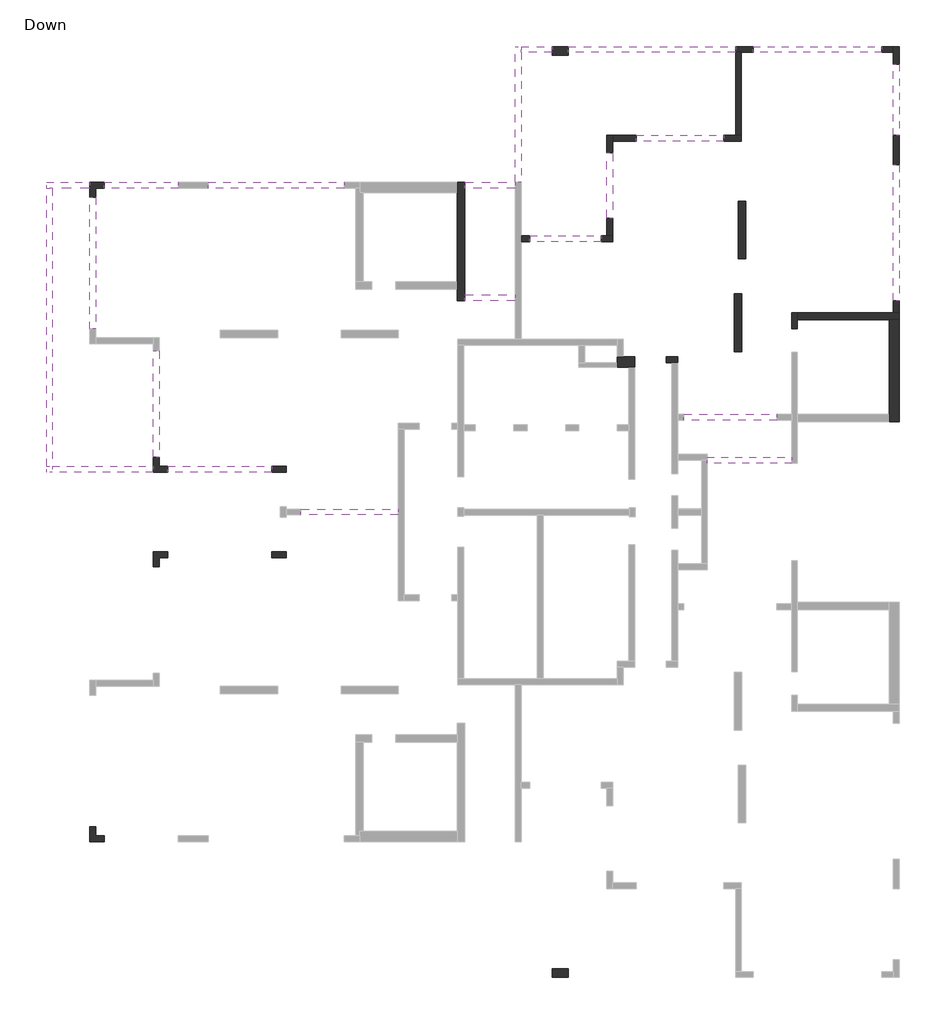
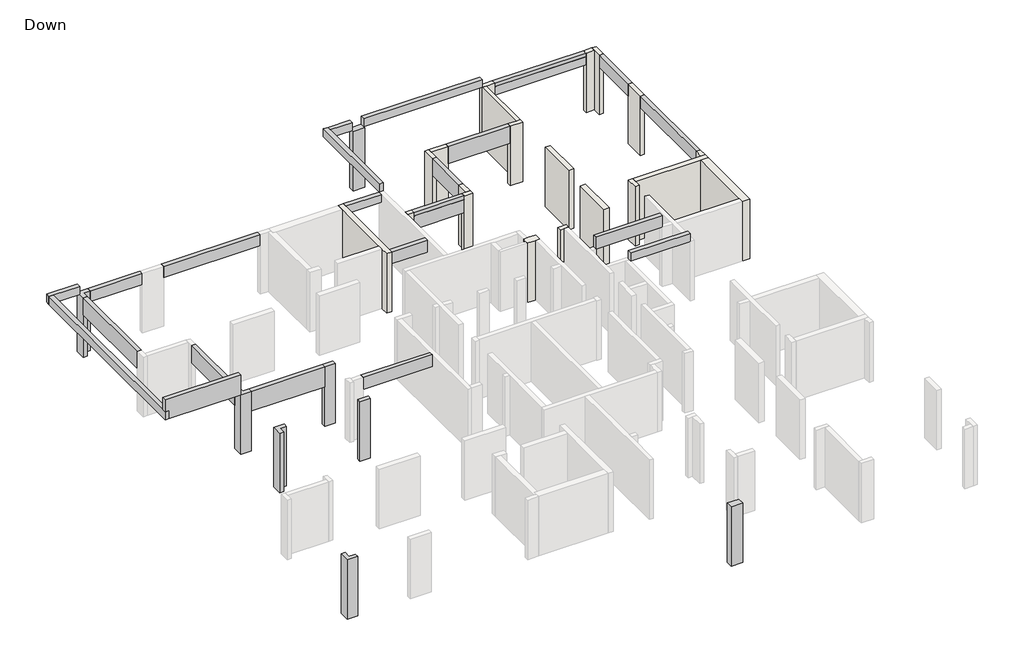
# One storey, part 3 of 3: 22 beams, 20 walls, 8 columns.
"""IFC4 building model written with IfcOpenShell, lengths in millimetres."""

from ifc_helpers import new_model, si_unit, frame, origin, place, context, project, spatial, polyline, outline, extrude, faceted_brep, element, save

model = new_model("IFC4")

# Units and contexts
model_context = context("Model", 3, world=origin())
ifc_project = project(units=[si_unit("LENGTHUNIT", "METRE", prefix="MILLI")], contexts=[model_context])

# Site, building, storey
site = spatial("IfcSite", under=ifc_project)
building = spatial("IfcBuilding", under=site)
storey = spatial("IfcBuildingStorey", under=building, Name="Down", Elevation=0.0)

# Beams
placement = place(None, origin())
element("IfcBeam", 1, ObjectType="Concrete Rectengular Beam : 20/40", at=placement, inside=storey, context=model_context, shape_type="Brep", body=[
    faceted_brep([(2246.4257984, 14641.4166181, 3400.0), (2246.4257984, 14641.4166181, 3000.0), (2446.4257984, 14641.4166181, 3000.0), (2446.4257984, 14641.4166181, 3400.0), (2446.4257984, 19040.9991377, 3400.0), (2446.4257984, 19240.9991377, 3400.0), (2246.4257984, 19240.9991377, 3400.0), (2446.4257984, 19040.9991377, 3000.0), (2446.4257984, 19240.9991377, 3000.0), (2246.4257984, 19240.9991377, 3000.0)], [[[0, 1, 2, 3]], [[0, 3, 4, 5, 6]], [[3, 2, 7, 8, 5, 4]], [[2, 1, 9, 8, 7]], [[1, 0, 6, 9]], [[6, 5, 8, 9]]]),
])
element("IfcBeam", 2, ObjectType="Concrete Rectengular Beam : 20/40", at=placement, inside=storey, context=model_context, shape_type="SweptSolid", body=[
    extrude(outline(polyline([(3495.6958179, 19240.9991377), (3495.6958179, 19040.9991377), (2446.4257984, 19040.9991377), (2446.4257984, 19240.9991377), (3495.6958179, 19240.9991377)])), frame((0.0, 0.0, 3000.0), z_axis=(0.0, 0.0, 1.0), x_axis=(1.0, 0.0, 0.0)), (0.0, 0.0, 1.0), 400.0),
])
element("IfcBeam", 3, ObjectType="Concrete Rectengular Beam : 20/40", at=placement, inside=storey, context=model_context, shape_type="SweptSolid", body=[
    extrude(outline(polyline([(9702.4292163, 19241.3311689), (9702.4292163, 19041.3311689), (4045.6958179, 19041.3311689), (4045.6958179, 19241.3311689), (9702.4292163, 19241.3311689)])), frame((0.0, 0.0, 3000.0), z_axis=(0.0, 0.0, 1.0), x_axis=(1.0, 0.0, 0.0)), (0.0, 0.0, 1.0), 400.0),
])
element("IfcBeam", 4, ObjectType="Concrete Rectengular Beam : 20/40", at=placement, inside=storey, context=model_context, shape_type="Brep", body=[
    faceted_brep([(2246.4257984, 14441.4166181, 3000.0), (2246.4257984, 14641.4166181, 3000.0), (542.9516773, 14641.4166181, 3000.0), (542.9516773, 14441.4166181, 3000.0), (2246.4257984, 14641.4166181, 2600.0), (542.9516773, 14641.4166181, 2600.0), (2246.4257984, 14441.4166181, 2600.0), (542.9516773, 14441.4166181, 2600.0), (2246.4257984, 14441.4166181, 2820.0), (542.9516773, 14441.4166181, 2820.0)], [[[0, 1, 2, 3]], [[1, 4, 5, 2]], [[4, 6, 7, 5]], [[6, 8, 0, 3, 9, 7]], [[1, 0, 8, 6, 4]], [[3, 2, 5, 7, 9]]]),
])
element("IfcBeam", 5, ObjectType="Concrete Rectengular Beam : 20/40", at=placement, inside=storey, context=model_context, shape_type="Brep", body=[
    faceted_brep([(-12154.2455884, 14441.4166181, 3400.0), (-12154.2455884, 14441.4166181, 3000.0), (-12154.2455884, 14641.4166181, 3000.0), (-12154.2455884, 14641.4166181, 3400.0), (-13614.2455884, 14641.4166181, 3400.0), (-13614.2455884, 14441.4166181, 3400.0), (-13414.2455884, 14441.4166181, 3400.0), (-13614.2455884, 14641.4166181, 3000.0), (-13414.2455884, 14441.4166181, 3000.0), (-13614.2455884, 14441.4166181, 3000.0)], [[[0, 1, 2, 3]], [[0, 3, 4, 5, 6]], [[3, 2, 7, 4]], [[2, 1, 8, 9, 7]], [[1, 0, 6, 5, 9, 8]], [[5, 4, 7, 9]]]),
])
element("IfcBeam", 6, ObjectType="Concrete Rectengular Beam : 20/40", at=placement, inside=storey, context=model_context, shape_type="Brep", body=[
    faceted_brep([(-13614.2455884, 4839.8443525, 3400.0), (-13414.2455884, 4839.8443525, 3400.0), (-13414.2455884, 5039.8443525, 3400.0), (-13414.2455884, 14441.4166181, 3400.0), (-13614.2455884, 14441.4166181, 3400.0), (-13614.2455884, 5039.8443525, 3400.0), (-13614.2455884, 4839.8443525, 3000.0), (-13614.2455884, 14441.4166181, 3000.0), (-13414.2455884, 4839.8443525, 3000.0), (-13414.2455884, 14441.4166181, 3000.0), (-13414.2455884, 5039.8443525, 3000.0)], [[[0, 1, 2, 3, 4, 5]], [[6, 0, 5, 4, 7]], [[8, 6, 7, 9, 10]], [[1, 8, 10, 9, 3, 2]], [[4, 3, 9, 7]], [[1, 0, 6, 8]]]),
])
element("IfcBeam", 7, ObjectType="Concrete Rectengular Beam : 20/40", at=placement, inside=storey, context=model_context, shape_type="SweptSolid", body=[
    extrude(outline(polyline([(8750.5859546, 5134.8297041), (8750.5859546, 5334.8297041), (11596.5527515, 5334.8297041), (11596.5527515, 5134.8297041), (8750.5859546, 5134.8297041)])), frame((0.0, 0.0, 3000.0), z_axis=(0.0, 0.0, 1.0), x_axis=(1.0, 0.0, 0.0)), (0.0, 0.0, 1.0), 400.0),
])
element("IfcBeam", 8, ObjectType="Concrete Rectengular Beam : 20/55", at=placement, inside=storey, context=model_context, shape_type="SweptSolid", body=[
    extrude(outline(polyline([(-11654.2455884, 14441.4166181), (-11654.2455884, 14641.4166181), (-9154.7387524, 14641.4166181), (-9154.7387524, 14441.4166181), (-11654.2455884, 14441.4166181)])), frame((0.0, 0.0, 2450.0), z_axis=(0.0, 0.0, 1.0), x_axis=(1.0, 0.0, 0.0)), (0.0, 0.0, 1.0), 550.0),
])
element("IfcBeam", 9, ObjectType="Concrete Rectengular Beam : 20/55", at=placement, inside=storey, context=model_context, shape_type="SweptSolid", body=[
    extrude(outline(polyline([(-3547.0483227, 14641.4166181), (-3547.0483227, 14441.4166181), (-8149.7387524, 14441.4166181), (-8149.7387524, 14641.4166181), (-3547.0483227, 14641.4166181)])), frame((0.0, 0.0, 2450.0), z_axis=(0.0, 0.0, 1.0), x_axis=(1.0, 0.0, 0.0)), (0.0, 0.0, 1.0), 550.0),
])
element("IfcBeam", 10, ObjectType="Concrete Rectengular Beam : 20/60", at=placement, inside=storey, context=model_context, shape_type="SweptSolid", body=[
    extrude(outline(polyline([(15047.1826343, 18641.3311689), (15247.1826343, 18641.3311689), (15247.1826343, 16232.3272627), (15047.1826343, 16232.3272627), (15047.1826343, 18641.3311689)])), frame((0.0, 0.0, 2400.0), z_axis=(0.0, 0.0, 1.0), x_axis=(1.0, 0.0, 0.0)), (0.0, 0.0, 1.0), 600.0),
])
element("IfcBeam", 11, ObjectType="Concrete Rectengular Beam : 20/60", at=placement, inside=storey, context=model_context, shape_type="SweptSolid", body=[
    extrude(outline(polyline([(15047.1826343, 15240.4498212), (15247.1826343, 15240.4498212), (15247.1826343, 10634.8394697), (15047.1826343, 10634.8394697), (15047.1826343, 15240.4498212)])), frame((0.0, 0.0, 2400.0), z_axis=(0.0, 0.0, 1.0), x_axis=(1.0, 0.0, 0.0)), (0.0, 0.0, 1.0), 600.0),
])
element("IfcBeam", 12, ObjectType="Concrete Rectengular Beam : 20/60", at=placement, inside=storey, context=model_context, shape_type="Brep", body=[
    faceted_brep([(2246.4257984, 10641.3507002, 3000.0), (2246.4257984, 10841.3507002, 3000.0), (542.9516773, 10841.3507002, 3000.0), (542.9516773, 10641.3507002, 3000.0), (2246.4257984, 10841.3507002, 2820.0), (2246.4257984, 10841.3507002, 2400.0), (542.9516773, 10841.3507002, 2400.0), (542.9516773, 10841.3507002, 2820.0), (2246.4257984, 10641.3507002, 2400.0), (542.9516773, 10641.3507002, 2400.0), (2246.4257984, 10641.3507002, 2820.0)], [[[0, 1, 2, 3]], [[1, 4, 5, 6, 7, 2]], [[5, 8, 9, 6]], [[8, 10, 0, 3, 9]], [[1, 0, 10, 8, 5, 4]], [[3, 2, 7, 6, 9]]]),
])
element("IfcBeam", 13, ObjectType="Concrete Rectengular Beam : 20/60", at=placement, inside=storey, context=model_context, shape_type="Brep", body=[
    faceted_brep([(-1704.8486157, 3390.0103681, 3000.0), (-1704.8486157, 3590.0103681, 3000.0), (-5004.9145337, 3590.0103681, 3000.0), (-5004.9145337, 3390.0103681, 3000.0), (-1704.8486157, 3390.0103681, 2400.0), (-1704.8486157, 3390.0103681, 2820.0), (-5004.9145337, 3390.0103681, 2400.0), (-1704.8486157, 3590.0103681, 2400.0), (-5004.9145337, 3590.0103681, 2400.0), (-1704.8486157, 3590.0103681, 2820.0)], [[[0, 1, 2, 3]], [[4, 5, 0, 3, 6]], [[7, 4, 6, 8]], [[1, 9, 7, 8, 2]], [[1, 0, 5, 4, 7, 9]], [[3, 2, 8, 6]]]),
])
element("IfcBeam", 14, ObjectType="Concrete Rectengular Beam : 20/60", at=placement, inside=storey, context=model_context, shape_type="SweptSolid", body=[
    extrude(outline(polyline([(11103.869646, 6791.3653486), (11103.869646, 6591.3653486), (7955.5859546, 6591.3653486), (7955.5859546, 6791.3653486), (11103.869646, 6791.3653486)])), frame((0.0, 0.0, 3000.0), z_axis=(0.0, 0.0, 1.0), x_axis=(1.0, 0.0, 0.0)), (0.0, 0.0, 1.0), 600.0),
])
element("IfcBeam", 15, ObjectType="Concrete Rectengular Beam : 20/60", at=placement, inside=storey, context=model_context, shape_type="SweptSolid", body=[
    extrude(outline(polyline([(19241.3311689, 2400.0), (19041.3311689, 2400.0), (19041.3311689, 2820.0), (19046.3311689, 2820.0), (19046.3311689, 3000.0), (19241.3311689, 3000.0), (19241.3311689, 2400.0)])), frame((10302.4292163, 0.0, 0.0), z_axis=(1.0, 0.0, 0.0), x_axis=(0.0, 1.0, 0.0)), (0.0, 0.0, 1.0), 4350.0610352),
])
element("IfcBeam", 16, ObjectType="Concrete Rectengular Beam : 20/85", at=placement, inside=storey, context=model_context, shape_type="Brep", body=[
    faceted_brep([(-11954.2455884, 14141.4166181, 3000.0), (-12154.2455884, 14141.4166181, 3000.0), (-12154.2455884, 9686.3702314, 3000.0), (-11954.2455884, 9686.3702314, 3000.0), (-11954.2455884, 14141.4166181, 2150.0), (-11954.2455884, 9686.3702314, 2150.0), (-12154.2455884, 14141.4166181, 2150.0), (-12154.2455884, 9686.3702314, 2150.0), (-12154.2455884, 14141.4166181, 2750.0), (-12154.2455884, 9686.3702314, 2750.0)], [[[0, 1, 2, 3]], [[4, 0, 3, 5]], [[6, 4, 5, 7]], [[2, 1, 8, 6, 7, 9]], [[1, 0, 4, 6, 8]], [[3, 2, 9, 7, 5]]]),
])
element("IfcBeam", 17, ObjectType="Concrete Rectengular Beam : 20/85", at=placement, inside=storey, context=model_context, shape_type="SweptSolid", body=[
    extrude(outline(polyline([(12840.2984541, 2150.0), (12640.2984541, 2150.0), (12640.2984541, 2820.0), (12645.2984541, 2820.0), (12645.2984541, 3000.0), (12840.2984541, 3000.0), (12840.2984541, 2150.0)])), frame((2745.6201343, 0.0, 0.0), z_axis=(1.0, 0.0, 0.0), x_axis=(0.0, 1.0, 0.0)), (0.0, 0.0, 1.0), 2406.9848633),
])
element("IfcBeam", 18, ObjectType="Concrete Rectengular Beam : 20/85", at=placement, inside=storey, context=model_context, shape_type="Brep", body=[
    faceted_brep([(5345.4492359, 13436.8389814, 3000.0), (5545.4492359, 13436.8389814, 3000.0), (5545.4492359, 15641.9757002, 3000.0), (5345.4492359, 15641.9757002, 3000.0), (5545.4492359, 13436.8389814, 2820.0), (5545.4492359, 13436.8389814, 2150.0), (5545.4492359, 15641.9757002, 2150.0), (5545.4492359, 15641.9757002, 2820.0), (5345.4492359, 13436.8389814, 2150.0), (5345.4492359, 15641.9757002, 2150.0), (5345.4492359, 15641.9757002, 2750.0), (5345.4492359, 13436.8389814, 2750.0)], [[[0, 1, 2, 3]], [[2, 1, 4, 5, 6, 7]], [[5, 8, 9, 6]], [[0, 3, 10, 9, 8, 11]], [[1, 0, 11, 8, 5, 4]], [[3, 2, 7, 6, 9, 10]]]),
])
element("IfcBeam", 19, ObjectType="Concrete Rectengular Beam : 20/85", at=placement, inside=storey, context=model_context, shape_type="Brep", body=[
    faceted_brep([(6350.1123218, 16241.9757002, 3000.0), (6350.1123218, 16041.9757002, 3000.0), (9302.4292163, 16041.9757002, 3000.0), (9302.4292163, 16241.9757002, 3000.0), (6350.1123218, 16041.9757002, 2820.0), (6350.1123218, 16041.9757002, 2150.0), (9302.4292163, 16041.9757002, 2150.0), (9302.4292163, 16041.9757002, 2820.0), (6350.1123218, 16241.9757002, 2150.0), (9302.4292163, 16241.9757002, 2150.0), (9302.4292163, 16241.9757002, 2750.0), (6350.1123218, 16241.9757002, 2750.0)], [[[0, 1, 2, 3]], [[2, 1, 4, 5, 6, 7]], [[5, 8, 9, 6]], [[0, 3, 10, 9, 8, 11]], [[1, 0, 11, 8, 5, 4]], [[3, 2, 7, 6, 9, 10]]]),
])
element("IfcBeam", 20, ObjectType="Concrete Rectengular Beam : 20/85", at=placement, inside=storey, context=model_context, shape_type="Brep", body=[
    faceted_brep([(-10005.5395337, 5339.8443525, 3000.0), (-9805.5395337, 5339.8443525, 3000.0), (-9805.5395337, 8939.7491377, 3000.0), (-10005.5395337, 8939.7491377, 3000.0), (-10005.5395337, 5339.8443525, 2150.0), (-10005.5395337, 8939.7491377, 2150.0), (-9805.5395337, 5339.8443525, 2150.0), (-9805.5395337, 8939.7491377, 2150.0), (-9805.5395337, 5339.8443525, 2820.0), (-9805.5395337, 8939.7491377, 2820.0)], [[[0, 1, 2, 3]], [[4, 0, 3, 5]], [[6, 4, 5, 7]], [[2, 1, 8, 6, 7, 9]], [[1, 0, 4, 6, 8]], [[3, 2, 9, 7, 5]]]),
])
element("IfcBeam", 21, ObjectType="Concrete Rectengular Beam : 25/100", at=placement, inside=storey, context=model_context, shape_type="SweptSolid", body=[
    extrude(outline(polyline([(3000.0, -10005.5395337), (4000.0, -10005.5395337), (4000.0, -13614.2455884), (3400.0, -13614.2455884), (3400.0, -13414.2455884), (3000.0, -13414.2455884), (3000.0, -10005.5395337)])), frame((0.0, 4839.8443525, 0.0), z_axis=(0.0, 1.0, 0.0), x_axis=(0.0, 0.0, 1.0)), (0.0, 0.0, 1.0), 200.0),
])
element("IfcBeam", 22, ObjectType="Concrete Rectengular Beam : 25/100", at=placement, inside=storey, context=model_context, shape_type="Brep", body=[
    faceted_brep([(-9505.5395337, 5039.8443525, 3000.0), (-9505.5395337, 4839.8443525, 3000.0), (-5999.4457837, 4839.8443525, 3000.0), (-5999.4457837, 5039.8443525, 3000.0), (-9505.5395337, 4839.8443525, 2000.0), (-5999.4457837, 4839.8443525, 2000.0), (-9505.5395337, 5039.8443525, 2000.0), (-5999.4457837, 5039.8443525, 2000.0), (-5999.4457837, 5039.8443525, 2820.0), (-9505.5395337, 5039.8443525, 2820.0)], [[[0, 1, 2, 3]], [[1, 4, 5, 2]], [[4, 6, 7, 5]], [[0, 3, 8, 7, 6, 9]], [[1, 0, 9, 6, 4]], [[3, 2, 5, 7, 8]]]),
])

# Columns
element("IfcColumn", 23, ObjectType="Concrete Rectengular Column : 20/50", at=placement, inside=storey, context=model_context, shape_type="Brep", body=[
    faceted_brep([(-5999.4457837, 5039.8443525, 0.0), (-5499.4457837, 5039.8443525, 0.0), (-5499.4457837, 4839.8443525, 0.0), (-5999.4457837, 4839.8443525, 0.0), (-5999.4457837, 5039.8443525, 3000.0), (-5499.4457837, 5039.8443525, 3000.0), (-5499.4457837, 5039.8443525, 2820.0), (-5499.4457837, 4839.8443525, 3000.0), (-5999.4457837, 4839.8443525, 3000.0)], [[[0, 1, 2, 3]], [[4, 5, 6, 1, 0]], [[5, 7, 2, 1, 6]], [[7, 8, 3, 2]], [[8, 4, 0, 3]], [[4, 8, 7, 5]]]),
])
element("IfcColumn", 24, ObjectType="Concrete Rectengular Column : 20/50", at=placement, inside=storey, context=model_context, shape_type="Brep", body=[
    faceted_brep([(-5999.4457837, 1940.1763837, 0.0), (-5999.4457837, 2140.1763837, 0.0), (-5499.4457837, 2140.1763837, 0.0), (-5499.4457837, 1940.1763837, 0.0), (-5999.4457837, 1940.1763837, 3000.0), (-5499.4457837, 1940.1763837, 2820.0), (-5499.4457837, 1940.1763837, 3000.0), (-5499.4457837, 2140.1763837, 3000.0), (-5999.4457837, 2140.1763837, 3000.0)], [[[0, 1, 2, 3]], [[4, 0, 3, 5, 6]], [[6, 5, 3, 2, 7]], [[7, 2, 1, 8]], [[8, 1, 0, 4]], [[4, 6, 7, 8]]]),
])
element("IfcColumn", 25, ObjectType="Concrete Rectengular Column : 30/55", at=placement, inside=storey, context=model_context, shape_type="Brep", body=[
    faceted_brep([(3495.6958179, 19240.9991377, 0.0), (4045.6958179, 19240.9991377, 0.0), (4045.6958179, 18940.9991377, 0.0), (3495.6958179, 18940.9991377, 0.0), (3495.6958179, 19240.9991377, 3000.0), (4045.6958179, 19240.9991377, 3000.0), (3495.6958179, 19240.9991377, 2750.0), (4045.6958179, 18940.9991377, 3000.0), (4045.6958179, 18940.9991377, 2750.0), (3495.6958179, 18940.9991377, 3000.0), (3495.6958179, 18940.9991377, 2750.0)], [[[0, 1, 2, 3]], [[4, 5, 1, 0, 6]], [[5, 7, 8, 2, 1]], [[7, 9, 10, 3, 2, 8]], [[9, 4, 6, 0, 3, 10]], [[4, 9, 7, 5]]]),
])
element("IfcColumn", 26, ObjectType="Concrete Rectengular Column : 30/55", at=placement, inside=storey, context=model_context, shape_type="Brep", body=[
    faceted_brep([(3495.6958179, -12260.9784014, 0.0), (3495.6958179, -11960.9784014, 0.0), (4045.6958179, -11960.9784014, 0.0), (4045.6958179, -12260.9784014, 0.0), (3495.6958179, -12260.9784014, 3000.0), (3495.6958179, -12260.9784014, 2750.0), (4045.6958179, -12260.9784014, 3000.0), (4045.6958179, -11960.9784014, 2750.0), (4045.6958179, -11960.9784014, 3000.0), (3495.6958179, -11960.9784014, 2750.0), (3495.6958179, -11960.9784014, 3000.0)], [[[0, 1, 2, 3]], [[4, 5, 0, 3, 6]], [[6, 3, 2, 7, 8]], [[8, 7, 2, 1, 9, 10]], [[10, 9, 1, 0, 5, 4]], [[4, 6, 8, 10]]]),
])
element("IfcColumn", 27, ObjectType="L Column : 50/50/20/20", at=placement, inside=storey, context=model_context, shape_type="Brep", body=[
    faceted_brep([(-12154.2455884, 14641.4166181, 0.0), (-11654.2455884, 14641.4166181, 0.0), (-11654.2455884, 14441.4166181, 0.0), (-11954.2455884, 14441.4166181, 0.0), (-11954.2455884, 14141.4166181, 0.0), (-12154.2455884, 14141.4166181, 0.0), (-12154.2455884, 14641.4166181, 3000.0), (-11654.2455884, 14641.4166181, 3000.0), (-12154.2455884, 14641.4166181, 2750.0), (-11654.2455884, 14441.4166181, 3000.0), (-11954.2455884, 14441.4166181, 3000.0), (-11954.2455884, 14441.4166181, 2820.0), (-11954.2455884, 14141.4166181, 3000.0), (-12154.2455884, 14141.4166181, 3000.0)], [[[0, 1, 2, 3, 4, 5]], [[6, 7, 1, 0, 8]], [[7, 9, 2, 1]], [[9, 10, 11, 3, 2]], [[10, 12, 4, 3, 11]], [[12, 13, 5, 4]], [[13, 6, 8, 0, 5]], [[6, 13, 12, 10, 9, 7]]]),
])
element("IfcColumn", 28, ObjectType="L Column : 50/50/20/20", at=placement, inside=storey, context=model_context, shape_type="Brep", body=[
    faceted_brep([(-10005.5395337, 4839.8443525, 0.0), (-10005.5395337, 5339.8443525, 0.0), (-9805.5395337, 5339.8443525, 0.0), (-9805.5395337, 5039.8443525, 0.0), (-9505.5395337, 5039.8443525, 0.0), (-9505.5395337, 4839.8443525, 0.0), (-10005.5395337, 4839.8443525, 3000.0), (-10005.5395337, 5339.8443525, 3000.0), (-10005.5395337, 4839.8443525, 2750.0), (-9805.5395337, 5339.8443525, 3000.0), (-9805.5395337, 5039.8443525, 3000.0), (-9805.5395337, 5039.8443525, 2820.0), (-9505.5395337, 5039.8443525, 3000.0), (-9505.5395337, 4839.8443525, 3000.0)], [[[0, 1, 2, 3, 4, 5]], [[6, 7, 1, 0, 8]], [[7, 9, 2, 1]], [[9, 10, 11, 3, 2]], [[10, 12, 4, 3, 11]], [[12, 13, 5, 4]], [[13, 6, 8, 0, 5]], [[6, 13, 12, 10, 9, 7]]]),
])
element("IfcColumn", 29, ObjectType="L Column : 50/50/20/20", at=placement, inside=storey, context=model_context, shape_type="Brep", body=[
    faceted_brep([(-12154.2455884, -7661.3958819, 0.0), (-12154.2455884, -7161.3958819, 0.0), (-11954.2455884, -7161.3958819, 0.0), (-11954.2455884, -7461.3958819, 0.0), (-11654.2455884, -7461.3958819, 0.0), (-11654.2455884, -7661.3958819, 0.0), (-12154.2455884, -7661.3958819, 3000.0), (-12154.2455884, -7661.3958819, 2750.0), (-11654.2455884, -7661.3958819, 3000.0), (-11654.2455884, -7461.3958819, 2820.0), (-11654.2455884, -7461.3958819, 3000.0), (-11654.2455884, -7466.3958819, 3000.0), (-11954.2455884, -7461.3958819, 2820.0), (-11954.2455884, -7461.3958819, 3000.0), (-11954.2455884, -7161.3958819, 3000.0), (-12154.2455884, -7161.3958819, 3000.0)], [[[0, 1, 2, 3, 4, 5]], [[6, 7, 0, 5, 8]], [[8, 5, 4, 9, 10, 11]], [[10, 9, 4, 3, 12, 13]], [[13, 12, 3, 2, 14]], [[14, 2, 1, 15]], [[15, 1, 0, 7, 6]], [[6, 8, 11, 10, 13, 14, 15]]]),
])
element("IfcColumn", 30, ObjectType="L Column : 50/50/20/20", at=placement, inside=storey, context=model_context, shape_type="Brep", body=[
    faceted_brep([(-10005.5395337, 2140.1763837, 0.0), (-9505.5395337, 2140.1763837, 0.0), (-9505.5395337, 1940.1763837, 0.0), (-9805.5395337, 1940.1763837, 0.0), (-9805.5395337, 1640.1763837, 0.0), (-10005.5395337, 1640.1763837, 0.0), (-10005.5395337, 2140.1763837, 3000.0), (-10005.5395337, 2140.1763837, 2750.0), (-10005.5395337, 1640.1763837, 3000.0), (-9805.5395337, 1640.1763837, 3000.0), (-9805.5395337, 1940.1763837, 2820.0), (-9805.5395337, 1940.1763837, 3000.0), (-9505.5395337, 1940.1763837, 3000.0), (-9505.5395337, 2140.1763837, 3000.0)], [[[0, 1, 2, 3, 4, 5]], [[6, 7, 0, 5, 8]], [[8, 5, 4, 9]], [[9, 4, 3, 10, 11]], [[11, 10, 3, 2, 12]], [[12, 2, 1, 13]], [[13, 1, 0, 7, 6]], [[6, 8, 9, 11, 12, 13]]]),
])

# Walls
element("IfcWall", 31, ObjectType="20", at=placement, inside=storey, context=model_context, shape_type="Brep", body=[
    faceted_brep([(2745.6201343, 12840.2984541, 0.0), (2446.4257984, 12840.2984541, 0.0), (2446.4257984, 12840.2984541, 3000.0), (2745.6201343, 12840.2984541, 3000.0), (2745.6201343, 12840.2984541, 2150.0), (2745.6201343, 12640.2984541, 0.0), (2745.6201343, 12640.2984541, 2150.0), (2745.6201343, 12640.2984541, 2820.0), (2745.6201343, 12640.2984541, 3000.0), (2446.4257984, 12640.2984541, 3000.0), (2446.4257984, 12640.2984541, 2820.0), (2446.4257984, 12640.2984541, 0.0), (2745.6201343, 12645.2984541, 3000.0)], [[[0, 1, 2, 3, 4]], [[5, 6, 7, 8, 9, 10, 11]], [[1, 0, 5, 11]], [[3, 2, 9, 8, 12]], [[0, 4, 3, 12, 8, 7, 6, 5]], [[2, 1, 11, 10, 9]]]),
])
element("IfcWall", 32, ObjectType="20", at=placement, inside=storey, context=model_context, shape_type="Brep", body=[
    faceted_brep([(5152.6049976, 12640.2984541, 0.0), (5545.4492359, 12640.2984541, 0.0), (5545.4492359, 12640.2984541, 2820.0), (5545.4492359, 12640.2984541, 3000.0), (5152.6049976, 12640.2984541, 3000.0), (5152.6049976, 12640.2984541, 2820.0), (5152.6049976, 12640.2984541, 2150.0), (5152.6049976, 12840.2984541, 0.0), (5152.6049976, 12840.2984541, 2150.0), (5152.6049976, 12840.2984541, 3000.0), (5345.4492359, 12840.2984541, 3000.0), (5545.4492359, 12840.2984541, 3000.0), (5545.4492359, 12840.2984541, 0.0), (5345.4492359, 12840.2984541, 0.0), (5152.6049976, 12645.2984541, 3000.0)], [[[0, 1, 2, 3, 4, 5, 6]], [[7, 8, 9, 10, 11, 12, 13]], [[1, 0, 7, 13, 12]], [[4, 3, 11, 10, 9, 14]], [[0, 6, 5, 4, 14, 9, 8, 7]], [[3, 2, 1, 12, 11]]]),
])
element("IfcWall", 33, ObjectType="20", at=placement, inside=storey, context=model_context, shape_type="Brep", body=[
    faceted_brep([(5545.4492359, 12840.2984541, 0.0), (5545.4492359, 13436.8389814, 0.0), (5545.4492359, 13436.8389814, 2150.0), (5545.4492359, 13436.8389814, 3000.0), (5545.4492359, 12840.2984541, 3000.0), (5345.4492359, 12840.2984541, 0.0), (5345.4492359, 12840.2984541, 2750.0), (5345.4492359, 12840.2984541, 3000.0), (5345.4492359, 13436.8389814, 3000.0), (5345.4492359, 13436.8389814, 2150.0), (5345.4492359, 13436.8389814, 0.0)], [[[0, 1, 2, 3, 4]], [[5, 6, 7, 8, 9, 10]], [[1, 0, 5, 10]], [[3, 2, 1, 10, 9, 8]], [[4, 3, 8, 7]], [[0, 4, 7, 6, 5]]]),
])
element("IfcWall", 34, ObjectType="20", at=placement, inside=storey, context=model_context, shape_type="Brep", body=[
    faceted_brep([(5545.4492359, 15641.9757002, 0.0), (5545.4492359, 16041.9757002, 0.0), (5545.4492359, 16241.9757002, 0.0), (5545.4492359, 16241.9757002, 3000.0), (5545.4492359, 16041.9757002, 3000.0), (5545.4492359, 15641.9757002, 3000.0), (5545.4492359, 15641.9757002, 2150.0), (5345.4492359, 15641.9757002, 0.0), (5345.4492359, 15641.9757002, 2150.0), (5345.4492359, 15641.9757002, 3000.0), (5345.4492359, 16241.9757002, 3000.0), (5345.4492359, 16241.9757002, 2750.0), (5345.4492359, 16241.9757002, 0.0)], [[[0, 1, 2, 3, 4, 5, 6]], [[7, 8, 9, 10, 11, 12]], [[2, 1, 0, 7, 12]], [[5, 4, 3, 10, 9]], [[0, 6, 5, 9, 8, 7]], [[3, 2, 12, 11, 10]]]),
])
element("IfcWall", 35, ObjectType="20", at=placement, inside=storey, context=model_context, shape_type="Brep", body=[
    faceted_brep([(5545.4492359, 16041.9757002, 0.0), (6350.1123218, 16041.9757002, 0.0), (6350.1123218, 16041.9757002, 2150.0), (6350.1123218, 16041.9757002, 3000.0), (5545.4492359, 16041.9757002, 3000.0), (5545.4492359, 16041.9757002, 2820.0), (5545.4492359, 16241.9757002, 0.0), (5545.4492359, 16241.9757002, 3000.0), (6350.1123218, 16241.9757002, 3000.0), (6350.1123218, 16241.9757002, 2150.0), (6350.1123218, 16241.9757002, 0.0)], [[[0, 1, 2, 3, 4, 5]], [[6, 7, 8, 9, 10]], [[1, 0, 6, 10]], [[3, 2, 1, 10, 9, 8]], [[4, 3, 8, 7]], [[0, 5, 4, 7, 6]]]),
])
element("IfcWall", 36, ObjectType="20", at=placement, inside=storey, context=model_context, shape_type="Brep", body=[
    faceted_brep([(9302.4292163, 16041.9561689, 0.0), (9902.4292163, 16041.9561689, 0.0), (9902.4292163, 16041.9561689, 2820.0), (9902.4292163, 16041.9561689, 3000.0), (9302.4292163, 16041.9561689, 3000.0), (9302.4292163, 16241.9561689, 0.0), (9302.4292163, 16241.9561689, 3000.0), (9702.4292163, 16241.9561689, 3000.0), (9902.4292163, 16241.9561689, 3000.0), (9902.4292163, 16241.9561689, 0.0), (9702.4292163, 16241.9561689, 0.0)], [[[0, 1, 2, 3, 4]], [[5, 6, 7, 8, 9, 10]], [[1, 0, 5, 10, 9]], [[4, 3, 8, 7, 6]], [[0, 4, 6, 5]], [[3, 2, 1, 9, 8]]]),
])
element("IfcWall", 37, ObjectType="20", at=placement, inside=storey, context=model_context, shape_type="Brep", body=[
    faceted_brep([(9902.4292163, 16241.9561689, 0.0), (9902.4292163, 19041.3311689, 0.0), (9902.4292163, 19041.3311689, 2820.0), (9902.4292163, 19041.3311689, 3000.0), (9902.4292163, 16241.9561689, 3000.0), (9702.4292163, 16241.9561689, 0.0), (9702.4292163, 16241.9561689, 2750.0), (9702.4292163, 16241.9561689, 3000.0), (9702.4292163, 19041.3311689, 3000.0), (9702.4292163, 19041.3311689, 0.0)], [[[0, 1, 2, 3, 4]], [[5, 6, 7, 8, 9]], [[1, 0, 5, 9]], [[4, 3, 8, 7]], [[0, 4, 7, 6, 5]], [[3, 2, 1, 9, 8]]]),
])
element("IfcWall", 38, ObjectType="20", at=placement, inside=storey, context=model_context, shape_type="Brep", body=[
    faceted_brep([(9702.4292163, 19041.3311689, 0.0), (9902.4292163, 19041.3311689, 0.0), (10302.4292163, 19041.3311689, 0.0), (10302.4292163, 19041.3311689, 2400.0), (10302.4292163, 19041.3311689, 2820.0), (10302.4292163, 19041.3311689, 3000.0), (9902.4292163, 19041.3311689, 3000.0), (9702.4292163, 19041.3311689, 3000.0), (9702.4292163, 19241.3311689, 0.0), (9702.4292163, 19241.3311689, 3000.0), (10302.4292163, 19241.3311689, 3000.0), (10302.4292163, 19241.3311689, 2400.0), (10302.4292163, 19241.3311689, 0.0), (10302.4292163, 19046.3311689, 3000.0)], [[[0, 1, 2, 3, 4, 5, 6, 7]], [[8, 9, 10, 11, 12]], [[2, 1, 0, 8, 12]], [[5, 4, 3, 2, 12, 11, 10, 13]], [[7, 6, 5, 13, 10, 9]], [[0, 7, 9, 8]]]),
])
element("IfcWall", 39, ObjectType="20", at=placement, inside=storey, context=model_context, shape_type="Brep", body=[
    faceted_brep([(14652.4902515, 19041.3311689, 0.0), (15047.1826343, 19041.3311689, 0.0), (15047.1826343, 19041.3311689, 2820.0), (15047.1826343, 19041.3311689, 3000.0), (14652.4902515, 19041.3311689, 3000.0), (14652.4902515, 19041.3311689, 2820.0), (14652.4902515, 19041.3311689, 2400.0), (14652.4902515, 19241.3311689, 0.0), (14652.4902515, 19241.3311689, 2400.0), (14652.4902515, 19241.3311689, 3000.0), (15047.1826343, 19241.3311689, 3000.0), (15047.1826343, 19241.3311689, 0.0), (14652.4902515, 19046.3311689, 3000.0)], [[[0, 1, 2, 3, 4, 5, 6]], [[7, 8, 9, 10, 11]], [[1, 0, 7, 11]], [[4, 3, 10, 9, 12]], [[0, 6, 5, 4, 12, 9, 8, 7]], [[3, 2, 1, 11, 10]]]),
])
element("IfcWall", 40, ObjectType="20", at=placement, inside=storey, context=model_context, shape_type="Brep", body=[
    faceted_brep([(15047.1826343, 19241.3311689, 0.0), (15047.1826343, 19041.3311689, 0.0), (15047.1826343, 18641.3311689, 0.0), (15047.1826343, 18641.3311689, 2400.0), (15047.1826343, 18641.3311689, 3000.0), (15047.1826343, 19041.3311689, 3000.0), (15047.1826343, 19241.3311689, 3000.0), (15247.1826343, 19241.3311689, 0.0), (15247.1826343, 19241.3311689, 3000.0), (15247.1826343, 18641.3311689, 3000.0), (15247.1826343, 18641.3311689, 2400.0), (15247.1826343, 18641.3311689, 0.0)], [[[0, 1, 2, 3, 4, 5, 6]], [[7, 8, 9, 10, 11]], [[2, 1, 0, 7, 11]], [[4, 3, 2, 11, 10, 9]], [[6, 5, 4, 9, 8]], [[0, 6, 8, 7]]]),
])
element("IfcWall", 41, ObjectType="20", at=placement, inside=storey, context=model_context, shape_type="Brep", body=[
    faceted_brep([(15047.1826343, 16232.3272627, 0.0), (15047.1826343, 15240.4498212, 0.0), (15047.1826343, 15240.4498212, 2400.0), (15047.1826343, 15240.4498212, 3000.0), (15047.1826343, 16232.3272627, 3000.0), (15047.1826343, 16232.3272627, 2400.0), (15247.1826343, 16232.3272627, 0.0), (15247.1826343, 16232.3272627, 2400.0), (15247.1826343, 16232.3272627, 3000.0), (15247.1826343, 15240.4498212, 3000.0), (15247.1826343, 15240.4498212, 2400.0), (15247.1826343, 15240.4498212, 0.0)], [[[0, 1, 2, 3, 4, 5]], [[6, 7, 8, 9, 10, 11]], [[1, 0, 6, 11]], [[3, 2, 1, 11, 10, 9]], [[4, 3, 9, 8]], [[0, 5, 4, 8, 7, 6]]]),
])
element("IfcWall", 42, ObjectType="20", at=placement, inside=storey, context=model_context, shape_type="Brep", body=[
    faceted_brep([(15047.1826343, 10634.8394697, 0.0), (15047.1826343, 10239.8248212, 0.0), (15047.1826343, 10239.8248212, 2820.0), (15047.1826343, 10239.8248212, 3000.0), (15047.1826343, 10634.8394697, 3000.0), (15047.1826343, 10634.8394697, 2400.0), (15247.1826343, 10634.8394697, 0.0), (15247.1826343, 10634.8394697, 2400.0), (15247.1826343, 10634.8394697, 3000.0), (15247.1826343, 10239.8248212, 3000.0), (15247.1826343, 10239.8248212, 0.0)], [[[0, 1, 2, 3, 4, 5]], [[6, 7, 8, 9, 10]], [[1, 0, 6, 10]], [[4, 3, 9, 8]], [[0, 5, 4, 8, 7, 6]], [[3, 2, 1, 10, 9]]]),
])
element("IfcWall", 43, ObjectType="20", at=placement, inside=storey, context=model_context, shape_type="Brep", body=[
    faceted_brep([(11596.5527515, 10239.8248212, 0.0), (11596.5527515, 9690.7110517, 0.0), (11596.5527515, 9690.7110517, 3000.0), (11596.5527515, 10239.8248212, 3000.0), (11596.5527515, 10239.8248212, 2820.0), (11796.5527515, 10239.8248212, 0.0), (11796.5527515, 10239.8248212, 3000.0), (11796.5527515, 9989.8248212, 3000.0), (11796.5527515, 9690.7110517, 3000.0), (11796.5527515, 9690.7110517, 0.0), (11796.5527515, 9989.8248212, 0.0)], [[[0, 1, 2, 3, 4]], [[5, 6, 7, 8, 9, 10]], [[1, 0, 5, 10, 9]], [[2, 1, 9, 8]], [[3, 2, 8, 7, 6]], [[0, 4, 3, 6, 5]]]),
])
element("IfcWall", 44, ObjectType="20", at=placement, inside=storey, context=model_context, shape_type="Brep", body=[
    faceted_brep([(7351.2304859, 8540.3936689, 0.0), (7551.2304859, 8540.3936689, 0.0), (7751.2304859, 8540.3936689, 0.0), (7751.2304859, 8540.3936689, 3000.0), (7551.2304859, 8540.3936689, 3000.0), (7351.2304859, 8540.3936689, 3000.0), (7351.2304859, 8540.3936689, 2820.0), (7351.2304859, 8740.3936689, 0.0), (7351.2304859, 8740.3936689, 2820.0), (7351.2304859, 8740.3936689, 3000.0), (7751.2304859, 8740.3936689, 3000.0), (7751.2304859, 8740.3936689, 2820.0), (7751.2304859, 8740.3936689, 0.0), (7351.2304859, 8739.7491377, 3000.0)], [[[0, 1, 2, 3, 4, 5, 6]], [[7, 8, 9, 10, 11, 12]], [[2, 1, 0, 7, 12]], [[5, 4, 3, 10, 9, 13]], [[0, 6, 5, 13, 9, 8, 7]], [[3, 2, 12, 11, 10]]]),
])
element("IfcWall", 45, ObjectType="25", at=placement, inside=storey, context=model_context, shape_type="Brep", body=[
    faceted_brep([(542.9516773, 10641.3507002, 0.0), (542.9516773, 14641.4166181, 0.0), (542.9516773, 14641.4166181, 2600.0), (542.9516773, 14641.4166181, 3000.0), (542.9516773, 14441.4166181, 3000.0), (542.9516773, 10841.3507002, 3000.0), (542.9516773, 10641.3507002, 3000.0), (292.9516773, 10641.3507002, 0.0), (292.9516773, 10641.3507002, 2820.0), (292.9516773, 10641.3507002, 3000.0), (292.9516773, 11035.7061689, 3000.0), (292.9516773, 11285.7061689, 3000.0), (292.9516773, 14291.4166181, 3000.0), (292.9516773, 14641.4166181, 3000.0), (292.9516773, 14641.4166181, 0.0), (292.9516773, 14291.4166181, 0.0), (292.9516773, 11285.7061689, 0.0), (292.9516773, 11035.7061689, 0.0)], [[[0, 1, 2, 3, 4, 5, 6]], [[7, 8, 9, 10, 11, 12, 13, 14, 15, 16, 17]], [[1, 0, 7, 17, 16, 15, 14]], [[6, 5, 4, 3, 13, 12, 11, 10, 9]], [[0, 6, 9, 8, 7]], [[3, 2, 1, 14, 13]]]),
])
element("IfcWall", 46, ObjectType="25", at=placement, inside=storey, context=model_context, shape_type="Brep", body=[
    faceted_brep([(9796.8798999, 14005.4864423, 0.0), (9796.8798999, 12062.9693525, 0.0), (9796.8798999, 12062.9693525, 2820.0), (9796.8798999, 12062.9693525, 3000.0), (9796.8798999, 14005.4864423, 3000.0), (9796.8798999, 14005.4864423, 2820.0), (10046.8798999, 14005.4864423, 0.0), (10046.8798999, 14005.4864423, 2820.0), (10046.8798999, 14005.4864423, 3000.0), (10046.8798999, 12062.9693525, 3000.0), (10046.8798999, 12062.9693525, 2820.0), (10046.8798999, 12062.9693525, 0.0)], [[[0, 1, 2, 3, 4, 5]], [[6, 7, 8, 9, 10, 11]], [[1, 0, 6, 11]], [[3, 2, 1, 11, 10, 9]], [[4, 3, 9, 8]], [[0, 5, 4, 8, 7, 6]]]),
])
element("IfcWall", 47, ObjectType="25", at=placement, inside=storey, context=model_context, shape_type="Brep", body=[
    faceted_brep([(9656.2060718, 10871.4141767, 0.0), (9656.2060718, 8920.2154462, 0.0), (9656.2060718, 8920.2154462, 2820.0), (9656.2060718, 8920.2154462, 3000.0), (9656.2060718, 10871.4141767, 3000.0), (9656.2060718, 10871.4141767, 2820.0), (9906.2060718, 10871.4141767, 0.0), (9906.2060718, 10871.4141767, 2820.0), (9906.2060718, 10871.4141767, 3000.0), (9906.2060718, 8920.2154462, 3000.0), (9906.2060718, 8920.2154462, 2820.0), (9906.2060718, 8920.2154462, 0.0)], [[[0, 1, 2, 3, 4, 5]], [[6, 7, 8, 9, 10, 11]], [[1, 0, 6, 11]], [[3, 2, 1, 11, 10, 9]], [[4, 3, 9, 8]], [[0, 5, 4, 8, 7, 6]]]),
])
element("IfcWall", 48, ObjectType="25", at=placement, inside=storey, context=model_context, shape_type="Brep", body=[
    faceted_brep([(11796.5527515, 9989.8248212, 0.0), (14897.1826343, 9989.8248212, 0.0), (15247.1826343, 9989.8248212, 0.0), (15247.1826343, 9989.8248212, 3000.0), (14897.1826343, 9989.8248212, 3000.0), (11796.5527515, 9989.8248212, 3000.0), (11796.5527515, 9989.8248212, 2820.0), (11796.5527515, 10239.8248212, 0.0), (11796.5527515, 10239.8248212, 3000.0), (15047.1826343, 10239.8248212, 3000.0), (15247.1826343, 10239.8248212, 3000.0), (15247.1826343, 10239.8248212, 0.0), (15047.1826343, 10239.8248212, 0.0)], [[[0, 1, 2, 3, 4, 5, 6]], [[7, 8, 9, 10, 11, 12]], [[2, 1, 0, 7, 12, 11]], [[5, 4, 3, 10, 9, 8]], [[3, 2, 11, 10]], [[0, 6, 5, 8, 7]]]),
])
element("IfcWall", 49, ObjectType="35", at=placement, inside=storey, context=model_context, shape_type="Brep", body=[
    faceted_brep([(14897.1826343, 9989.8248212, 0.0), (14897.1826343, 6791.445915, 0.0), (14897.1826343, 6541.445915, 0.0), (14897.1826343, 6541.445915, 3000.0), (14897.1826343, 6791.445915, 3000.0), (14897.1826343, 9989.8248212, 3000.0), (14897.1826343, 9989.8248212, 2820.0), (15247.1826343, 9989.8248212, 0.0), (15247.1826343, 9989.8248212, 3000.0), (15247.1826343, 6541.445915, 3000.0), (15247.1826343, 6541.445915, 0.0)], [[[0, 1, 2, 3, 4, 5, 6]], [[7, 8, 9, 10]], [[2, 1, 0, 7, 10]], [[5, 4, 3, 9, 8]], [[0, 6, 5, 8, 7]], [[3, 2, 10, 9]]]),
])
element("IfcWall", 50, ObjectType="35", at=placement, inside=storey, context=model_context, shape_type="Brep", body=[
    faceted_brep([(6296.4111499, 8740.0714033, 0.0), (5901.4257984, 8740.0714033, 0.0), (5701.4257984, 8740.0714033, 0.0), (5701.4257984, 8740.0714033, 3000.0), (5901.4257984, 8740.0714033, 3000.0), (6296.4111499, 8740.0714033, 3000.0), (6296.4111499, 8740.0714033, 2820.0), (6296.4111499, 8390.0714033, 0.0), (6296.4111499, 8390.0714033, 3000.0), (6096.4111499, 8390.0714033, 3000.0), (5701.4257984, 8390.0714033, 3000.0), (5701.4257984, 8390.0714033, 0.0), (6096.4111499, 8390.0714033, 0.0), (5701.4257984, 8540.0714033, 0.0), (5701.4257984, 8540.0714033, 3000.0), (6296.4111499, 8739.7491377, 3000.0)], [[[0, 1, 2, 3, 4, 5, 6]], [[7, 8, 9, 10, 11, 12]], [[2, 1, 0, 7, 12, 11, 13]], [[5, 4, 3, 14, 10, 9, 8, 15]], [[3, 2, 13, 11, 10, 14]], [[0, 6, 5, 15, 8, 7]]]),
])

save(model, "model.ifc")

# Revit data of these elements
# Type "Concrete Rectengular Beam : 20/40"
#   Keynote = "09000"
#   Length [instance default] = 152.4 cm
#   b = 20 cm
#   h = 40 cm
#   Structural Material [instance default] = Concrete
#   Assembly Code = ""
# Type "Concrete Rectengular Beam : 20/55"
#   Length [instance default] = 152.4 cm
#   b = 20 cm
#   h = 55 cm
#   Structural Material [instance default] = Concrete
#   Assembly Code = ""
# Type "Concrete Rectengular Beam : 20/60"
#   Length [instance default] = 152.4 cm
#   b = 20 cm
#   h = 60 cm
#   Structural Material [instance default] = Concrete
#   Assembly Code = ""
# Type "Concrete Rectengular Beam : 20/85"
#   Length [instance default] = 152.4 cm
#   b = 20 cm
#   h = 85 cm
#   Structural Material [instance default] = Concrete
#   Assembly Code = ""
# Type "Concrete Rectengular Beam : 25/100"
#   Length [instance default] = 152.4 cm
#   b = 20 cm
#   h = 100 cm
#   Structural Material [instance default] = Concrete
#   Assembly Code = ""
# Type "Concrete Rectengular Column : 20/50"
#   b = 20 cm
#   h = 50 cm
#   Structural Material [instance default] = Concrete
# Type "Concrete Rectengular Column : 30/55"
#   b = 30 cm
#   h = 55 cm
#   Structural Material [instance default] = Concrete
# Type "L Column : 50/50/20/20"
#   Small Length = 20 cm
#   Small Depth = 20 cm
#   Depth = 50 cm
#   Length = 50 cm
#   Centroid Y = 70 cm
#   Centroid X = 10 cm
#   Structural Material [instance default] = Concrete, Cast-in-Place gray
# Type "20"
#   Layers, outside or top first: 20 cm "Concrete" (function 1)
# Type "25"
#   Layers, outside or top first: 25 cm "Concrete" (function 1)
# Type "35"
#   Layers, outside or top first: 35 cm "Concrete" (function 1)
# Element 1 (IfcBeam, "Concrete Rectengular Beam : 20/40")
#   Comments = ""
#   Mark = "B1"
#   SOFiSTiK_AMG_Comments = ""
#   SOFiSTiK_AMG_Scheduled = yes
#   SOFiSTiK_AMG_Adjusted = yes
#   Structural Material = Concrete
#   Phase Created = New Construction
#   Materials on its faces: "Concrete"
# Element 2 (IfcBeam, "Concrete Rectengular Beam : 20/40")
#   Comments = ""
#   Mark = "B2"
#   SOFiSTiK_AMG_Comments = ""
#   SOFiSTiK_AMG_Scheduled = yes
#   SOFiSTiK_AMG_Adjusted = yes
#   Structural Material = Concrete
#   Phase Created = New Construction
#   Materials on its faces: "Concrete"
# Element 3 (IfcBeam, "Concrete Rectengular Beam : 20/40")
#   Comments = ""
#   Mark = "B3"
#   SOFiSTiK_AMG_Comments = ""
#   SOFiSTiK_AMG_Scheduled = yes
#   SOFiSTiK_AMG_Adjusted = yes
#   Structural Material = Concrete
#   Phase Created = New Construction
#   Materials on its faces: "Concrete"
# Element 4 (IfcBeam, "Concrete Rectengular Beam : 20/40")
#   Comments = ""
#   Mark = "B4"
#   SOFiSTiK_AMG_Comments = ""
#   SOFiSTiK_AMG_Scheduled = yes
#   SOFiSTiK_AMG_Adjusted = yes
#   Structural Material = Concrete
#   Phase Created = New Construction
#   Materials on its faces: "Concrete"
# Element 5 (IfcBeam, "Concrete Rectengular Beam : 20/40")
#   Comments = ""
#   Mark = "B5"
#   SOFiSTiK_AMG_Comments = ""
#   SOFiSTiK_AMG_Scheduled = yes
#   SOFiSTiK_AMG_Adjusted = yes
#   Structural Material = Concrete
#   Phase Created = New Construction
#   Materials on its faces: "Concrete"
# Element 6 (IfcBeam, "Concrete Rectengular Beam : 20/40")
#   Comments = ""
#   Mark = "B6"
#   SOFiSTiK_AMG_Comments = ""
#   SOFiSTiK_AMG_Scheduled = yes
#   SOFiSTiK_AMG_Adjusted = yes
#   Structural Material = Concrete
#   Phase Created = New Construction
#   Materials on its faces: "Concrete"
# Element 7 (IfcBeam, "Concrete Rectengular Beam : 20/40")
#   Comments = ""
#   Mark = "B7"
#   SOFiSTiK_AMG_Comments = ""
#   SOFiSTiK_AMG_Scheduled = yes
#   SOFiSTiK_AMG_Adjusted = yes
#   Structural Material = Concrete
#   Phase Created = New Construction
#   Materials on its faces: "Concrete"
# Element 8 (IfcBeam, "Concrete Rectengular Beam : 20/55")
#   Comments = ""
#   Mark = "B15"
#   SOFiSTiK_AMG_Comments = ""
#   SOFiSTiK_AMG_Scheduled = yes
#   SOFiSTiK_AMG_Adjusted = yes
#   Structural Material = Concrete
#   Phase Created = New Construction
#   Materials on its faces: "Concrete"
# Element 9 (IfcBeam, "Concrete Rectengular Beam : 20/55")
#   Comments = ""
#   Mark = "B16"
#   SOFiSTiK_AMG_Comments = ""
#   SOFiSTiK_AMG_Scheduled = yes
#   SOFiSTiK_AMG_Adjusted = yes
#   Structural Material = Concrete
#   Phase Created = New Construction
#   Materials on its faces: "Concrete"
# Element 10 (IfcBeam, "Concrete Rectengular Beam : 20/60")
#   Comments = ""
#   Mark = "B19"
#   SOFiSTiK_AMG_Comments = ""
#   SOFiSTiK_AMG_Scheduled = yes
#   SOFiSTiK_AMG_Adjusted = yes
#   Structural Material = Concrete
#   Phase Created = New Construction
#   Materials on its faces: "Concrete"
# Element 11 (IfcBeam, "Concrete Rectengular Beam : 20/60")
#   Comments = ""
#   Mark = "B20"
#   SOFiSTiK_AMG_Comments = ""
#   SOFiSTiK_AMG_Scheduled = yes
#   SOFiSTiK_AMG_Adjusted = yes
#   Structural Material = Concrete
#   Phase Created = New Construction
#   Materials on its faces: "Concrete"
# Element 12 (IfcBeam, "Concrete Rectengular Beam : 20/60")
#   Comments = ""
#   Mark = "B21"
#   SOFiSTiK_AMG_Comments = ""
#   SOFiSTiK_AMG_Scheduled = yes
#   SOFiSTiK_AMG_Adjusted = yes
#   Structural Material = Concrete
#   Phase Created = New Construction
#   Materials on its faces: "Concrete"
# Element 13 (IfcBeam, "Concrete Rectengular Beam : 20/60")
#   Comments = ""
#   Mark = "B22"
#   SOFiSTiK_AMG_Comments = ""
#   SOFiSTiK_AMG_Scheduled = yes
#   SOFiSTiK_AMG_Adjusted = yes
#   Structural Material = Concrete
#   Phase Created = New Construction
#   Materials on its faces: "Concrete"
# Element 14 (IfcBeam, "Concrete Rectengular Beam : 20/60")
#   Comments = ""
#   Mark = "B23"
#   SOFiSTiK_AMG_Comments = ""
#   SOFiSTiK_AMG_Scheduled = yes
#   SOFiSTiK_AMG_Adjusted = yes
#   Structural Material = Concrete
#   Phase Created = New Construction
#   Materials on its faces: "Concrete"
# Element 15 (IfcBeam, "Concrete Rectengular Beam : 20/60")
#   Comments = ""
#   Mark = "B24"
#   SOFiSTiK_AMG_Comments = ""
#   SOFiSTiK_AMG_Scheduled = yes
#   SOFiSTiK_AMG_Adjusted = yes
#   Structural Material = Concrete
#   Phase Created = New Construction
#   Materials on its faces: "Concrete"
# Element 16 (IfcBeam, "Concrete Rectengular Beam : 20/85")
#   Comments = ""
#   Mark = "B30"
#   SOFiSTiK_AMG_Comments = ""
#   SOFiSTiK_AMG_Scheduled = yes
#   SOFiSTiK_AMG_Adjusted = yes
#   Structural Material = Concrete
#   Phase Created = New Construction
#   Materials on its faces: "Concrete"
# Element 17 (IfcBeam, "Concrete Rectengular Beam : 20/85")
#   Comments = ""
#   Mark = "B31"
#   SOFiSTiK_AMG_Comments = ""
#   SOFiSTiK_AMG_Scheduled = yes
#   SOFiSTiK_AMG_Adjusted = yes
#   Structural Material = Concrete
#   Phase Created = New Construction
#   Materials on its faces: "Concrete"
# Element 18 (IfcBeam, "Concrete Rectengular Beam : 20/85")
#   Comments = ""
#   Mark = "B32"
#   SOFiSTiK_AMG_Comments = ""
#   SOFiSTiK_AMG_Scheduled = yes
#   SOFiSTiK_AMG_Adjusted = yes
#   Structural Material = Concrete
#   Phase Created = New Construction
#   Materials on its faces: "Concrete"
# Element 19 (IfcBeam, "Concrete Rectengular Beam : 20/85")
#   Comments = ""
#   Mark = "B33"
#   SOFiSTiK_AMG_Comments = ""
#   SOFiSTiK_AMG_Scheduled = yes
#   SOFiSTiK_AMG_Adjusted = yes
#   Structural Material = Concrete
#   Phase Created = New Construction
#   Materials on its faces: "Concrete"
# Element 20 (IfcBeam, "Concrete Rectengular Beam : 20/85")
#   Comments = ""
#   Mark = "B34"
#   SOFiSTiK_AMG_Comments = ""
#   SOFiSTiK_AMG_Scheduled = yes
#   SOFiSTiK_AMG_Adjusted = yes
#   Structural Material = Concrete
#   Phase Created = New Construction
#   Materials on its faces: "Concrete"
# Element 21 (IfcBeam, "Concrete Rectengular Beam : 25/100")
#   Comments = ""
#   Mark = "B40"
#   SOFiSTiK_AMG_Comments = ""
#   SOFiSTiK_AMG_Scheduled = yes
#   SOFiSTiK_AMG_Adjusted = yes
#   Structural Material = Concrete
#   Phase Created = New Construction
#   Materials on its faces: "Concrete"
# Element 22 (IfcBeam, "Concrete Rectengular Beam : 25/100")
#   Comments = ""
#   Mark = "B41"
#   SOFiSTiK_AMG_Comments = ""
#   SOFiSTiK_AMG_Scheduled = yes
#   SOFiSTiK_AMG_Adjusted = yes
#   Structural Material = Concrete
#   Phase Created = New Construction
#   Materials on its faces: "Concrete"
# Element 23 (IfcColumn, "Concrete Rectengular Column : 20/50")
#   Comments = ""
#   Mark = "C1"
#   SOFiSTiK_AMG_Comments = ""
#   SOFiSTiK_AMG_Scheduled = yes
#   SOFiSTiK_AMG_Adjusted = yes
#   Structural Material = Concrete
#   Phase Created = New Construction
#   Materials on its faces: "Concrete"
# Element 24 (IfcColumn, "Concrete Rectengular Column : 20/50")
#   Comments = ""
#   Mark = "C2"
#   SOFiSTiK_AMG_Comments = ""
#   SOFiSTiK_AMG_Scheduled = yes
#   SOFiSTiK_AMG_Adjusted = yes
#   Structural Material = Concrete
#   Phase Created = New Construction
#   Materials on its faces: "Concrete"
# Element 25 (IfcColumn, "Concrete Rectengular Column : 30/55")
#   Comments = ""
#   Mark = "C3"
#   SOFiSTiK_AMG_Comments = ""
#   SOFiSTiK_AMG_Scheduled = yes
#   SOFiSTiK_AMG_Adjusted = yes
#   Structural Material = Concrete
#   Phase Created = New Construction
#   Materials on its faces: "Concrete"
# Element 26 (IfcColumn, "Concrete Rectengular Column : 30/55")
#   Comments = ""
#   Mark = "C4"
#   SOFiSTiK_AMG_Comments = ""
#   SOFiSTiK_AMG_Scheduled = yes
#   SOFiSTiK_AMG_Adjusted = yes
#   Structural Material = Concrete
#   Phase Created = New Construction
#   Materials on its faces: "Concrete"
# Element 27 (IfcColumn, "L Column : 50/50/20/20")
#   Comments = ""
#   Mark = "C5"
#   SOFiSTiK_AMG_Comments = ""
#   SOFiSTiK_AMG_Scheduled = yes
#   SOFiSTiK_AMG_Adjusted = yes
#   Structural Material = Concrete
#   Phase Created = New Construction
# Element 28 (IfcColumn, "L Column : 50/50/20/20")
#   Comments = ""
#   Mark = "C6"
#   SOFiSTiK_AMG_Comments = ""
#   SOFiSTiK_AMG_Scheduled = yes
#   SOFiSTiK_AMG_Adjusted = yes
#   Structural Material = Concrete
#   Phase Created = New Construction
# Element 29 (IfcColumn, "L Column : 50/50/20/20")
#   Comments = ""
#   Mark = "C7"
#   SOFiSTiK_AMG_Comments = ""
#   SOFiSTiK_AMG_Scheduled = yes
#   SOFiSTiK_AMG_Adjusted = yes
#   Structural Material = Concrete
#   Phase Created = New Construction
# Element 30 (IfcColumn, "L Column : 50/50/20/20")
#   Comments = ""
#   Mark = "C8"
#   SOFiSTiK_AMG_Comments = ""
#   SOFiSTiK_AMG_Scheduled = yes
#   SOFiSTiK_AMG_Adjusted = yes
#   Structural Material = Concrete
#   Phase Created = New Construction
# Element 31 (IfcWall, "20")
#   Comments = ""
#   Mark = "W7"
#   SOFiSTiK_EdgeZones = "W7"
#   SOFiSTiK_AMG_Comments = ""
#   Top Offset = 0 cm
#   Base Offset = 0 cm
#   wall height = 300 cm
#   SOFiSTiK_AMG_Scheduled = yes
#   SOFiSTiK_AMG_Adjusted = yes
#   Phase Created = New Construction
#   Base Constraint = Down
#   Top Constraint = Typical Floor
#   Materials on its faces: "Concrete"
# Element 32 (IfcWall, "20")
#   Comments = ""
#   Mark = "W8"
#   SOFiSTiK_EdgeZones = "W8"
#   SOFiSTiK_AMG_Comments = ""
#   Top Offset = 0 cm
#   Base Offset = 0 cm
#   wall height = 300 cm
#   SOFiSTiK_AMG_Scheduled = yes
#   SOFiSTiK_AMG_Adjusted = yes
#   Phase Created = New Construction
#   Base Constraint = Down
#   Top Constraint = Typical Floor
#   Materials on its faces: "Concrete"
# Element 33 (IfcWall, "20")
#   Comments = ""
#   Mark = "W9"
#   SOFiSTiK_EdgeZones = "W9"
#   SOFiSTiK_AMG_Comments = ""
#   Top Offset = 0 cm
#   Base Offset = 0 cm
#   wall height = 300 cm
#   SOFiSTiK_AMG_Scheduled = yes
#   SOFiSTiK_AMG_Adjusted = yes
#   Phase Created = New Construction
#   Base Constraint = Down
#   Top Constraint = Typical Floor
#   Materials on its faces: "Concrete"
# Element 34 (IfcWall, "20")
#   Comments = ""
#   Mark = "W10"
#   SOFiSTiK_EdgeZones = "W10"
#   SOFiSTiK_AMG_Comments = ""
#   Top Offset = 0 cm
#   Base Offset = 0 cm
#   wall height = 300 cm
#   SOFiSTiK_AMG_Scheduled = yes
#   SOFiSTiK_AMG_Adjusted = yes
#   Phase Created = New Construction
#   Base Constraint = Down
#   Top Constraint = Typical Floor
#   Materials on its faces: "Concrete"
# Element 35 (IfcWall, "20")
#   Comments = ""
#   Mark = "W11"
#   SOFiSTiK_EdgeZones = "W11"
#   SOFiSTiK_AMG_Comments = ""
#   Top Offset = 0 cm
#   Base Offset = 0 cm
#   wall height = 300 cm
#   SOFiSTiK_AMG_Scheduled = yes
#   SOFiSTiK_AMG_Adjusted = yes
#   Phase Created = New Construction
#   Base Constraint = Down
#   Top Constraint = Typical Floor
#   Materials on its faces: "Concrete"
# Element 36 (IfcWall, "20")
#   Comments = ""
#   Mark = "W12"
#   SOFiSTiK_EdgeZones = "W12"
#   SOFiSTiK_AMG_Comments = ""
#   Top Offset = 0 cm
#   Base Offset = 0 cm
#   wall height = 300 cm
#   SOFiSTiK_AMG_Scheduled = yes
#   SOFiSTiK_AMG_Adjusted = yes
#   Phase Created = New Construction
#   Base Constraint = Down
#   Top Constraint = Typical Floor
#   Materials on its faces: "Concrete"
# Element 37 (IfcWall, "20")
#   Comments = ""
#   Mark = "W13"
#   SOFiSTiK_EdgeZones = "W13"
#   SOFiSTiK_AMG_Comments = ""
#   Top Offset = 0 cm
#   Base Offset = 0 cm
#   wall height = 300 cm
#   SOFiSTiK_AMG_Scheduled = yes
#   SOFiSTiK_AMG_Adjusted = yes
#   Phase Created = New Construction
#   Base Constraint = Down
#   Top Constraint = Typical Floor
#   Materials on its faces: "Concrete"
# Element 38 (IfcWall, "20")
#   Comments = ""
#   Mark = "W14"
#   SOFiSTiK_EdgeZones = "W14"
#   SOFiSTiK_AMG_Comments = ""
#   Top Offset = 0 cm
#   Base Offset = 0 cm
#   wall height = 300 cm
#   SOFiSTiK_AMG_Scheduled = yes
#   SOFiSTiK_AMG_Adjusted = yes
#   Phase Created = New Construction
#   Base Constraint = Down
#   Top Constraint = Typical Floor
#   Materials on its faces: "Concrete"
# Element 39 (IfcWall, "20")
#   Comments = ""
#   Mark = "W15"
#   SOFiSTiK_EdgeZones = "W15"
#   SOFiSTiK_AMG_Comments = ""
#   Top Offset = 0 cm
#   Base Offset = 0 cm
#   wall height = 300 cm
#   SOFiSTiK_AMG_Scheduled = yes
#   SOFiSTiK_AMG_Adjusted = yes
#   Phase Created = New Construction
#   Base Constraint = Down
#   Top Constraint = Typical Floor
#   Materials on its faces: "Concrete"
# Element 40 (IfcWall, "20")
#   Comments = ""
#   Mark = "W16"
#   SOFiSTiK_EdgeZones = "W16"
#   SOFiSTiK_AMG_Comments = ""
#   Top Offset = 0 cm
#   Base Offset = 0 cm
#   wall height = 300 cm
#   SOFiSTiK_AMG_Scheduled = yes
#   SOFiSTiK_AMG_Adjusted = yes
#   Phase Created = New Construction
#   Base Constraint = Down
#   Top Constraint = Typical Floor
#   Materials on its faces: "Concrete"
# Element 41 (IfcWall, "20")
#   Comments = ""
#   Mark = "W17"
#   SOFiSTiK_EdgeZones = "W17"
#   SOFiSTiK_AMG_Comments = ""
#   Top Offset = 0 cm
#   Base Offset = 0 cm
#   wall height = 300 cm
#   SOFiSTiK_AMG_Scheduled = yes
#   SOFiSTiK_AMG_Adjusted = yes
#   Phase Created = New Construction
#   Base Constraint = Down
#   Top Constraint = Typical Floor
#   Materials on its faces: "Concrete"
# Element 42 (IfcWall, "20")
#   Comments = ""
#   Mark = "W18"
#   SOFiSTiK_EdgeZones = "W18"
#   SOFiSTiK_AMG_Comments = ""
#   Top Offset = 0 cm
#   Base Offset = 0 cm
#   wall height = 300 cm
#   SOFiSTiK_AMG_Scheduled = yes
#   SOFiSTiK_AMG_Adjusted = yes
#   Phase Created = New Construction
#   Base Constraint = Down
#   Top Constraint = Typical Floor
#   Materials on its faces: "Concrete"
# Element 43 (IfcWall, "20")
#   Comments = ""
#   Mark = "W19"
#   SOFiSTiK_EdgeZones = "W19"
#   SOFiSTiK_AMG_Comments = ""
#   Top Offset = 0 cm
#   Base Offset = 0 cm
#   wall height = 300 cm
#   SOFiSTiK_AMG_Scheduled = yes
#   SOFiSTiK_AMG_Adjusted = yes
#   Phase Created = New Construction
#   Base Constraint = Down
#   Top Constraint = Typical Floor
#   Materials on its faces: "Concrete"
# Element 44 (IfcWall, "20")
#   Comments = ""
#   Mark = "W33"
#   SOFiSTiK_EdgeZones = "W33"
#   SOFiSTiK_AMG_Comments = ""
#   Top Offset = 0 cm
#   Base Offset = 0 cm
#   wall height = 300 cm
#   SOFiSTiK_AMG_Scheduled = yes
#   SOFiSTiK_AMG_Adjusted = yes
#   Phase Created = New Construction
#   Base Constraint = Down
